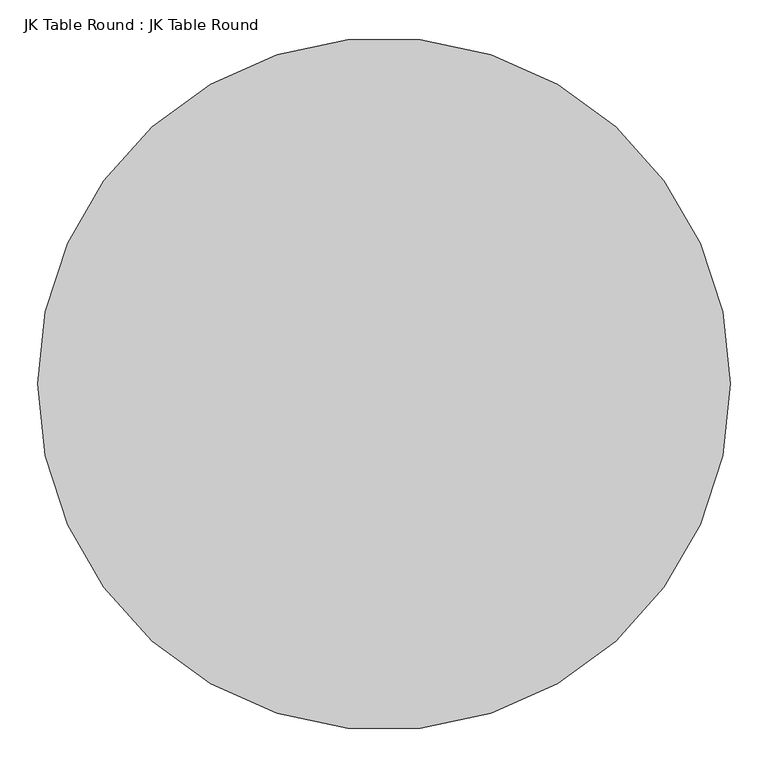
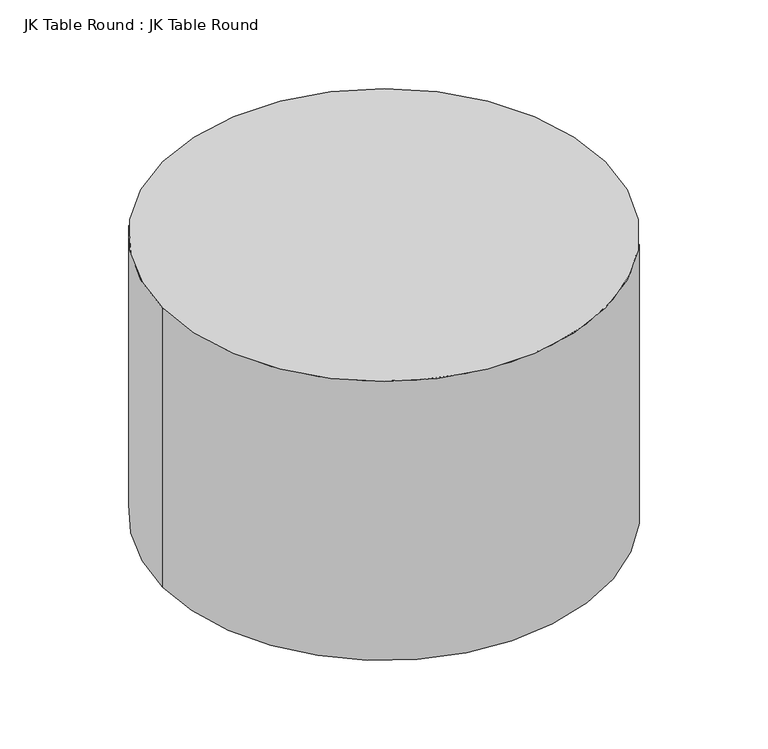
"""IFC4 building model written with IfcOpenShell, lengths in millimetres: furniture geometry, JK Table Round : JK Table Round."""

from ifc_helpers import new_model, si_unit, point, frame_2d, origin, origin_with_axes, place, context, project, spatial, circle_curve, trimmed, segment, composite_curve, outline, extrude, source, transform, mapped, element, save


def jk_table_round_jk_table_round_1ab66767(model_context):
    return source(origin(), model_context, "Body", "SweptSolid", [
        extrude(outline(composite_curve([segment(trimmed(circle_curve(frame_2d((-61.9426335, 33.5455296)), 457.2), [point((-519.1426335, 33.5455296))], [point((395.2573665, 33.5455296))], False, "CARTESIAN"), True, "CONTINUOUS"), segment(trimmed(circle_curve(frame_2d((-61.9426335, 33.5455296)), 457.2), [point((395.2573665, 33.5455296))], [point((-519.1426335, 33.5455296))], False, "CARTESIAN"), True, "CONTINUOUS")], self_intersect=False)), origin_with_axes(), (0.0, 0.0, 1.0), 609.6),
    ])


if __name__ == "__main__":
    model = new_model("IFC4")
    model_context = context("Model", 3, world=origin())
    ifc_project = project(units=[si_unit("LENGTHUNIT", "METRE", prefix="MILLI")], contexts=[model_context])
    site = spatial("IfcSite", under=ifc_project)
    building = spatial("IfcBuilding", under=site)
    placement = place(None, origin())
    jk_table_round_jk_table_round_shape = jk_table_round_jk_table_round_1ab66767(model_context)
    element("IfcFurniture", 1, ObjectType="JK Table Round : JK Table Round", at=placement, inside=building, context=model_context, shape_type="MappedRepresentation", body=[
        mapped(jk_table_round_jk_table_round_shape, transform((0.0, 0.0, 0.0), x_axis=(1.0, 0.0, 0.0), y_axis=(0.0, 1.0, 0.0), z_axis=(0.0, 0.0, 1.0))),
    ])
    save(model, "model.ifc")

# Revit data of these elements
# Type "JK Table Round : JK Table Round"
#   Width = 3' - 0"
#   Height = 2' - 0"
#   Status [instance default] = none
#   Default Elevation = 0
